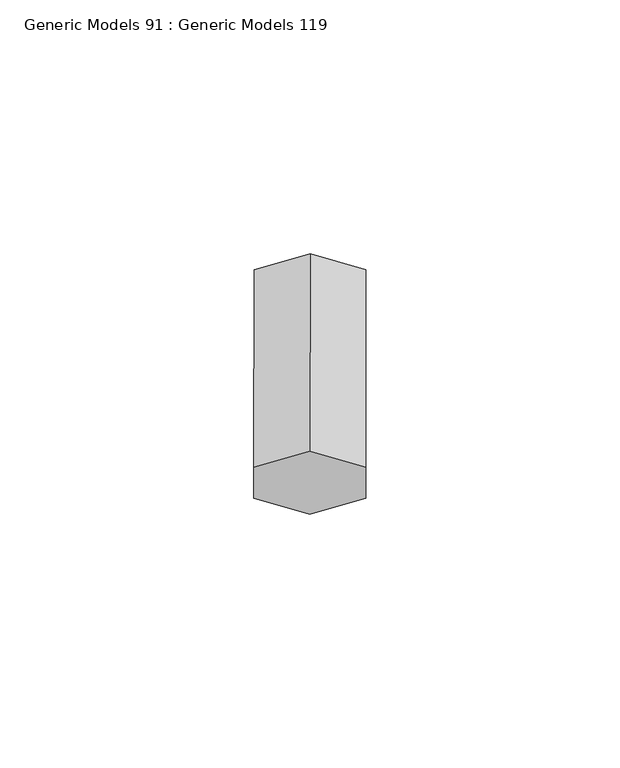
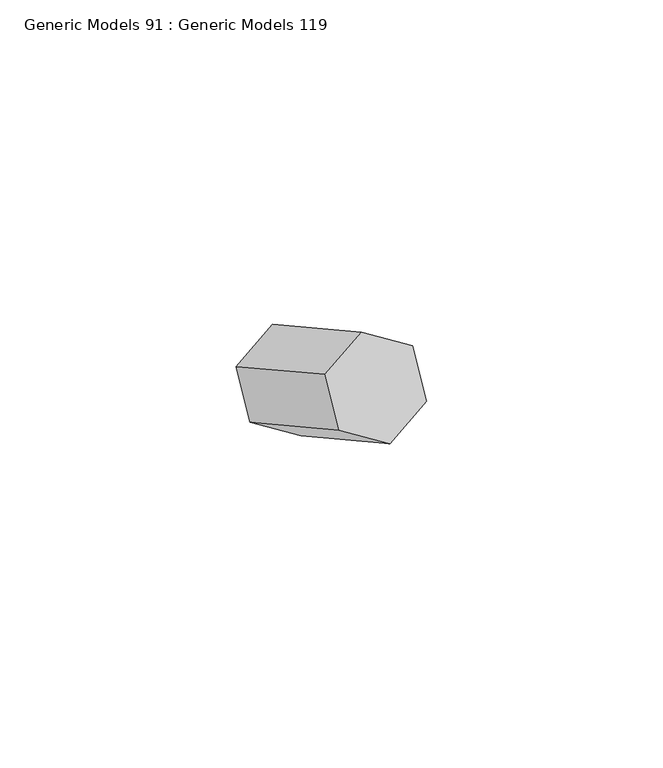
"""IFC4 building model written with IfcOpenShell, lengths in millimetres: proxy geometry, Generic Models 91 : Generic Models 119."""

from ifc_helpers import new_model, si_unit, origin, place, context, project, spatial, faceted_brep, source, transform, mapped, element, save


def generic_models_91_generic_models_119_ea17cf43(model_context):
    return source(origin(), model_context, "Body", "Brep", [
        faceted_brep([(31956.3469127, 35169.9910653, 269236.7040475), (31956.3469127, 35163.8339831, 269225.5963772), (31945.3483901, 35160.755442, 269220.0425421), (31934.3498675, 35163.8339831, 269225.5963772), (31934.3498675, 35169.9910653, 269236.7040475), (31945.3483901, 35173.0696064, 269242.2578827), (31956.2923001, 35131.1142193, 269258.2538351), (31945.2937775, 35134.1927604, 269263.8076703), (31934.2952549, 35131.1142193, 269258.2538351), (31934.2952549, 35124.9571371, 269247.1461649), (31945.2937775, 35121.878596, 269241.5923297), (31956.2923001, 35124.9571371, 269247.1461649)], [[[0, 1, 2, 3, 4, 5]], [[6, 7, 8, 9, 10, 11]], [[6, 11, 1, 0]], [[11, 10, 2, 1]], [[10, 9, 3, 2]], [[9, 8, 4, 3]], [[8, 7, 5, 4]], [[7, 6, 0, 5]]]),
    ])


if __name__ == "__main__":
    model = new_model("IFC4")
    model_context = context("Model", 3, world=origin())
    ifc_project = project(units=[si_unit("LENGTHUNIT", "METRE", prefix="MILLI")], contexts=[model_context])
    site = spatial("IfcSite", under=ifc_project)
    building = spatial("IfcBuilding", under=site)
    placement = place(None, origin())
    generic_models_91_generic_models_119_shape = generic_models_91_generic_models_119_ea17cf43(model_context)
    element("IfcBuildingElementProxy", 1, Name="Generic Models 91 : Generic Models 119", ObjectType="Generic Models 91 : Generic Models 119", at=placement, inside=building, context=model_context, shape_type="MappedRepresentation", body=[
        mapped(generic_models_91_generic_models_119_shape, transform((0.0, 0.0, 0.0), x_axis=(1.0, 0.0, 0.0), y_axis=(0.0, 1.0, 0.0), z_axis=(0.0, 0.0, 1.0))),
    ])
    save(model, "model.ifc")
